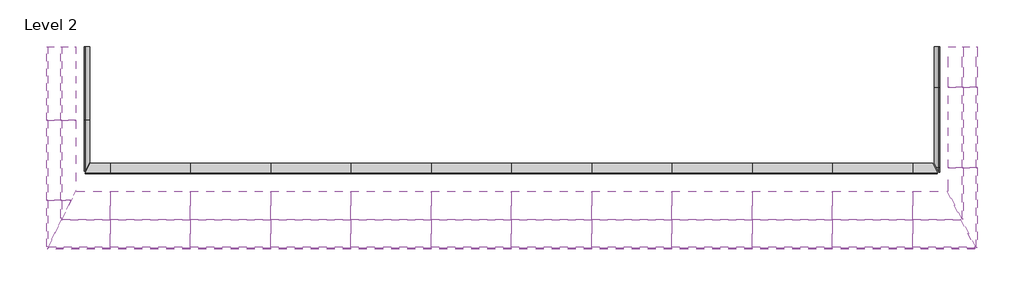
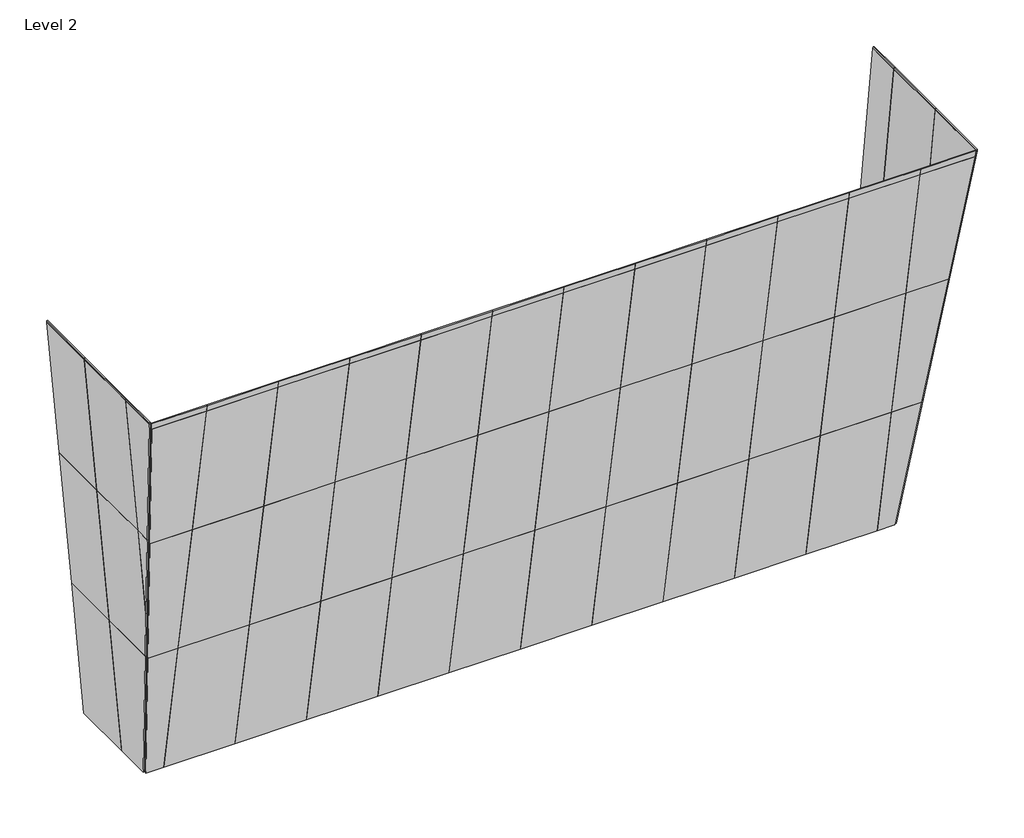
# One storey: 71 plates.
"""IFC4 building model written with IfcOpenShell, lengths in millimetres."""

import ifcopenshell
import ifcopenshell.guid

model = None  # the IFC model being written
_history = None  # IfcOwnerHistory: only IFC2X3 demands one
_inside = {}  # id of a spatial element -> (the spatial element, [elements in it])
_under = {}  # id of a project, library or spatial element -> (it, [spatial elements below it])
_declared = {}  # id of a project -> (the project, [libraries it declares])
_typed = {}  # id of a type object -> (the type object, [elements of that type])
_made_of = {}  # id of a material, layer set ... -> (it, [elements and type objects made of it])


def new_model(schema):
    """Start an empty IFC model of exactly this schema.

    Asked for "IFC4X3", IfcOpenShell would pick the latest addendum, in which some entities
    have other attributes; the version numbers below select the first issue.
    IFC2X3 requires an IfcOwnerHistory on every rooted entity: one is made here for all.
    """
    global model, _history
    if schema == "IFC4X3":
        model = ifcopenshell.file(schema_version=(4, 3, 0, 0))
    else:
        model = ifcopenshell.file(schema=schema)
    _inside.clear()
    _under.clear()
    _declared.clear()
    _typed.clear()
    _made_of.clear()
    _history = None
    if model.schema == "IFC2X3":
        org = make("IfcOrganization", Name="unknown")
        user = make(
            "IfcPersonAndOrganization",
            ThePerson=make("IfcPerson", FamilyName="unknown"),
            TheOrganization=org,
        )
        app = make(
            "IfcApplication",
            ApplicationDeveloper=org,
            Version="unknown",
            ApplicationFullName="unknown",
            ApplicationIdentifier="unknown",
        )
        _history = make(
            "IfcOwnerHistory",
            OwningUser=user,
            OwningApplication=app,
            ChangeAction="ADDED",
            CreationDate=0,
        )
    return model


def make(cls, **values):
    """One entity of the class cls with the attributes given. An attribute that is None is left unset."""
    return model.create_entity(
        cls, **{name: value for name, value in values.items() if value is not None}
    )


def rooted(cls, **values):
    """An entity with a GlobalId (a new one), such as an element, a storey or a relation."""
    return make(cls, GlobalId=ifcopenshell.guid.new(), OwnerHistory=_history, **values)


def si_unit(unit_type, name, prefix=None):
    """IfcSIUnit, for example si_unit("LENGTHUNIT", "METRE", prefix="MILLI")."""
    return make("IfcSIUnit", UnitType=unit_type, Prefix=prefix, Name=name)


def assignment(units):
    """IfcUnitAssignment: the units of a project."""
    return None if units is None else make("IfcUnitAssignment", Units=units)


def point(xyz):
    """IfcCartesianPoint."""
    return None if xyz is None else make("IfcCartesianPoint", Coordinates=xyz)


def direction(xyz):
    """IfcDirection."""
    return None if xyz is None else make("IfcDirection", DirectionRatios=xyz)


def frame(location, z_axis=None, x_axis=None):
    """IfcAxis2Placement3D, a coordinate frame: its origin and axes. An axis left out is left unset."""
    return make(
        "IfcAxis2Placement3D",
        Location=point(location),
        Axis=direction(z_axis),
        RefDirection=direction(x_axis),
    )


def origin():
    """The frame at (0, 0, 0) with its axes left unset."""
    return frame((0.0, 0.0, 0.0))


def origin_with_axes():
    """The frame at (0, 0, 0) with the z axis (0, 0, 1) and the x axis (1, 0, 0) written out."""
    return frame((0.0, 0.0, 0.0), z_axis=(0.0, 0.0, 1.0), x_axis=(1.0, 0.0, 0.0))


def place(relative_to, where):
    """IfcLocalPlacement: puts the frame where relative to a parent placement (None: the world)."""
    return make(
        "IfcLocalPlacement", PlacementRelTo=relative_to, RelativePlacement=where
    )


def context(
    kind, dimensions, precision=None, world=None, true_north=None, identifier=None
):
    """IfcGeometricRepresentationContext, for example the 3D "Model" context."""
    return make(
        "IfcGeometricRepresentationContext",
        ContextIdentifier=identifier,
        ContextType=kind,
        CoordinateSpaceDimension=dimensions,
        Precision=precision,
        WorldCoordinateSystem=world,
        TrueNorth=true_north,
    )


def project(units=None, contexts=None):
    """IfcProject with its units and contexts."""
    return rooted(
        "IfcProject",
        Name="project",
        RepresentationContexts=contexts,
        UnitsInContext=assignment(units),
    )


def spatial(cls, under=None, at=None, **own):
    """A site, building, storey or space (cls), placed at a placement, below another one or the project."""
    s = rooted(cls, ObjectPlacement=at, **own)
    if under is not None:
        _under.setdefault(under.id(), (under, []))[1].append(s)
    return s


def polyline(points):
    """IfcPolyline through the points."""
    return make("IfcPolyline", Points=[point(p) for p in points])


def outline(outer, holes=None, kind="AREA"):
    """IfcArbitraryClosedProfileDef: a profile drawn as a closed curve; with holes, ...WithVoids."""
    if holes is None:
        return make("IfcArbitraryClosedProfileDef", ProfileType=kind, OuterCurve=outer)
    return make(
        "IfcArbitraryProfileDefWithVoids",
        ProfileType=kind,
        OuterCurve=outer,
        InnerCurves=holes,
    )


def extrude(swept, where, along, depth):
    """IfcExtrudedAreaSolid: the profile swept, set in the frame where, extruded along a direction by depth."""
    return make(
        "IfcExtrudedAreaSolid",
        SweptArea=swept,
        Position=where,
        ExtrudedDirection=direction(along),
        Depth=depth,
    )


def shape(context_of_items, identifier, shape_type, items):
    """IfcShapeRepresentation: the items that make up one representation, for example the "Body"."""
    return make(
        "IfcShapeRepresentation",
        ContextOfItems=context_of_items,
        RepresentationIdentifier=identifier,
        RepresentationType=shape_type,
        Items=items,
    )


def source(mapping_origin, context_of_items, identifier, shape_type, items):
    """IfcRepresentationMap: a shape defined once, which mapped items show again and again."""
    return make(
        "IfcRepresentationMap",
        MappingOrigin=mapping_origin,
        MappedRepresentation=shape(context_of_items, identifier, shape_type, items),
    )


def transform(
    local_origin,
    x_axis=None,
    y_axis=None,
    z_axis=None,
    scale=None,
    scale2=None,
    scale3=None,
    uniform=True,
):
    """IfcCartesianTransformationOperator3D, or its non-uniform kind. x_axis, y_axis, z_axis: its Axis1, 2, 3."""
    if uniform:
        return make(
            "IfcCartesianTransformationOperator3D",
            Axis1=direction(x_axis),
            Axis2=direction(y_axis),
            LocalOrigin=point(local_origin),
            Scale=scale,
            Axis3=direction(z_axis),
        )
    return make(
        "IfcCartesianTransformationOperator3DnonUniform",
        Axis1=direction(x_axis),
        Axis2=direction(y_axis),
        LocalOrigin=point(local_origin),
        Scale=scale,
        Axis3=direction(z_axis),
        Scale2=scale2,
        Scale3=scale3,
    )


def mapped(mapping_source, mapping_target):
    """IfcMappedItem: shows the shape of a source again, moved by a transform."""
    return make(
        "IfcMappedItem", MappingSource=mapping_source, MappingTarget=mapping_target
    )


def made_of(thing, what):
    """Note that an element or type object is made of a material, layer set ...; save() writes the relation."""
    if what is not None:
        _made_of.setdefault(what.id(), (what, []))[1].append(thing)
    return thing


def element(
    cls,
    number,
    at=None,
    inside=None,
    cuts=None,
    type_object=None,
    material=None,
    context=None,
    identifier="Body",
    shape_type=None,
    held_by="IfcProductDefinitionShape",
    body=None,
    shapes=None,
    **own,
):
    """One element of the class cls, such as IfcWall. Its Tag is "e" and its number.

    at: its placement. inside: the storey or other place that contains it. cuts: it is an
    opening in that element (IfcRelVoidsElement). A single representation is given by context,
    identifier, shape_type and body (its items); several are given by shapes. held_by: the class
    of the entity that holds the representations. save() writes the other relations.
    """
    e = rooted(cls, Tag="e%d" % number, ObjectPlacement=at, **own)
    if body is not None:
        shapes = [shape(context, identifier, shape_type, body)]
    if shapes is not None:
        e.Representation = make(held_by, Representations=shapes)
    if inside is not None:
        _inside.setdefault(inside.id(), (inside, []))[1].append(e)
    if cuts is not None:
        rooted(
            "IfcRelVoidsElement", RelatingBuildingElement=cuts, RelatedOpeningElement=e
        )
    if type_object is not None:
        _typed.setdefault(type_object.id(), (type_object, []))[1].append(e)
    return made_of(e, material)


def aggregate(whole, parts):
    """IfcRelAggregates: a whole, such as a stair, and the parts it consists of."""
    return rooted("IfcRelAggregates", RelatingObject=whole, RelatedObjects=parts)


def save(model, path):
    """Write the relations noted so far, then the file.

    IfcRelAggregates (storeys below a building ...), IfcRelContainedInSpatialStructure (elements
    in a storey), IfcRelDefinesByType, IfcRelAssociatesMaterial and IfcRelDeclares: one each for
    every whole, place, type object, material and project.
    """
    for whole, parts in _under.values():
        aggregate(whole, parts)
    for where, things in _inside.values():
        rooted(
            "IfcRelContainedInSpatialStructure",
            RelatedElements=things,
            RelatingStructure=where,
        )
    for kind, things in _typed.values():
        rooted("IfcRelDefinesByType", RelatedObjects=things, RelatingType=kind)
    for what, things in _made_of.values():
        rooted("IfcRelAssociatesMaterial", RelatedObjects=things, RelatingMaterial=what)
    for by, libraries in _declared.values():
        rooted("IfcRelDeclares", RelatingContext=by, RelatedDefinitions=libraries)
    model.write(path)


def system_panel_glazed_2e91cb65(model_context):
    return source(origin(), model_context, "Body", "SweptSolid", [
        extrude(outline(polyline([(838.2000002, -44.45), (-838.2000002, -44.45), (-838.2000002, -19.05), (838.2000002, -19.05), (838.2000002, -44.45)])), origin_with_axes(), (0.0, 0.0, 1.0), 3657.6),
    ])


def system_panel_glazed_41c8569a(model_context):
    return source(origin(), model_context, "Body", "SweptSolid", [
        extrude(outline(polyline([(3054.1438606, -268.2393521), (0.0, 268.2393521), (3054.1438606, 268.2393521), (3054.1438606, -268.2393521)])), frame((0.0, -44.45, 0.0), z_axis=(0.0, 1.0, 0.0), x_axis=(0.0, 0.0, 1.0)), (0.0, 0.0, 1.0), 25.4),
    ])


def system_panel_glazed_2bad594a(model_context):
    return source(origin(), model_context, "Body", "SweptSolid", [
        extrude(outline(polyline([(0.0, -797.3917397), (0.0, 154.912342), (3657.6, 797.3917397), (3657.6, -797.3917397), (0.0, -797.3917397)])), frame((0.0, -44.45, 0.0), z_axis=(0.0, 1.0, 0.0), x_axis=(0.0, 0.0, 1.0)), (0.0, 0.0, 1.0), 25.4),
    ])


def system_panel_glazed_87679f4c(model_context):
    return source(origin(), model_context, "Body", "SweptSolid", [
        extrude(outline(polyline([(0.0, -914.4), (0.0, 680.3834794), (1332.2432262, 914.4), (3657.6, 914.4), (3657.6, -914.4), (0.0, -914.4)])), frame((0.0, -44.45, 0.0), z_axis=(0.0, 1.0, 0.0), x_axis=(0.0, 0.0, 1.0)), (0.0, 0.0, 1.0), 25.4),
    ])


def system_panel_glazed_96c5221b(model_context):
    return source(origin(), model_context, "Body", "SweptSolid", [
        extrude(outline(polyline([(0.0, -204.2314386), (2325.3567738, 204.2314386), (2325.3567738, -204.2314386), (0.0, -204.2314386)])), frame((0.0, -44.45, 0.0), z_axis=(0.0, 1.0, 0.0), x_axis=(0.0, 0.0, 1.0)), (0.0, 0.0, 1.0), 25.4),
    ])


def system_panel_glazed_1f34555f(model_context):
    return source(origin(), model_context, "Body", "SweptSolid", [
        extrude(outline(polyline([(914.4, -44.45), (-914.4, -44.45), (-914.4, -19.05), (914.4, -19.05), (914.4, -44.45)])), origin_with_axes(), (0.0, 0.0, 1.0), 3657.6),
    ])


def system_panel_glazed_ce152239(model_context):
    return source(origin(), model_context, "Body", "SweptSolid", [
        extrude(outline(polyline([(0.0, -525.4711374), (0.0, -117.0082603), (3657.6, 525.4711374), (3657.6, -525.4711374), (0.0, -525.4711374)])), frame((0.0, -44.45, 0.0), z_axis=(0.0, 1.0, 0.0), x_axis=(0.0, 0.0, 1.0)), (0.0, 0.0, 1.0), 25.4),
    ])


def system_panel_glazed_8b4ddac8(model_context):
    return source(origin(), model_context, "Body", "SweptSolid", [
        extrude(outline(polyline([(838.2000002, -44.45), (-838.2000002, -44.45), (-838.2000002, -19.05), (838.2000002, -19.05), (838.2000002, -44.45)])), origin_with_axes(), (0.0, 0.0, 1.0), 41.9143134),
    ])


def system_panel_glazed_7f82afe2(model_context):
    return source(origin(), model_context, "Body", "SweptSolid", [
        extrude(outline(polyline([(914.4, -44.45), (-914.4, -44.45), (-914.4, -19.05), (914.4, -19.05), (914.4, -44.45)])), origin_with_axes(), (0.0, 0.0, 1.0), 41.9143134),
    ])


def system_panel_glazed_3146f186(model_context):
    return source(origin(), model_context, "Body", "SweptSolid", [
        extrude(outline(polyline([(0.0, -529.1523878), (0.0, 521.789887), (41.9143134, 529.1523878), (41.9143134, -529.1523878), (0.0, -529.1523878)])), frame((0.0, -44.45, 0.0), z_axis=(0.0, 1.0, 0.0), x_axis=(0.0, 0.0, 1.0)), (0.0, 0.0, 1.0), 25.4),
    ])


def system_panel_glazed_f4345ae3(model_context):
    return source(origin(), model_context, "Body", "SweptSolid", [
        extrude(outline(polyline([(914.4, -44.45), (-914.4, -44.45), (-914.4, -19.05), (914.4, -19.05), (914.4, -44.45)])), origin_with_axes(), (0.0, 0.0, 1.0), 169.2731269),
    ])


def system_panel_glazed_866ab655(model_context):
    return source(origin(), model_context, "Body", "SweptSolid", [
        extrude(outline(polyline([(0.0, -808.3993064), (0.0, 914.4), (3657.6, 914.4), (3657.6, -914.4), (603.4561394, -914.4), (0.0, -808.3993064)])), frame((0.0, -44.45, 0.0), z_axis=(0.0, 1.0, 0.0), x_axis=(0.0, 0.0, 1.0)), (0.0, 0.0, 1.0), 25.4),
    ])


def system_panel_glazed_b062bbc2(model_context):
    return source(origin(), model_context, "Body", "SweptSolid", [
        extrude(outline(polyline([(465.8483058, -44.45), (-465.8483058, -44.45), (-465.8483058, -19.05), (465.8483058, -19.05), (465.8483058, -44.45)])), origin_with_axes(), (0.0, 0.0, 1.0), 3657.6),
    ])


def system_panel_glazed_bcd6892e(model_context):
    return source(origin(), model_context, "Body", "SweptSolid", [
        extrude(outline(polyline([(0.0, 53.0003468), (0.0, 589.4790509), (3657.6, 589.4790509), (3657.6, -589.4790509), (0.0, 53.0003468)])), frame((0.0, -44.45, 0.0), z_axis=(0.0, 1.0, 0.0), x_axis=(0.0, 0.0, 1.0)), (0.0, 0.0, 1.0), 25.4),
    ])


def system_panel_glazed_e7bd2299(model_context):
    return source(origin(), model_context, "Body", "SweptSolid", [
        extrude(outline(polyline([(0.0, -268.2393521), (0.0, 910.7187498), (3657.6, 910.7187498), (3657.6, -910.7187498), (0.0, -268.2393521)])), frame((0.0, -44.45, 0.0), z_axis=(0.0, 1.0, 0.0), x_axis=(0.0, 0.0, 1.0)), (0.0, 0.0, 1.0), 25.4),
    ])


def system_panel_glazed_0a43eb3e(model_context):
    return source(origin(), model_context, "Body", "SweptSolid", [
        extrude(outline(polyline([(0.0, -907.0374994), (0.0, 914.4000002), (41.9143134, 914.4000002), (41.9143134, -914.4000002), (0.0, -907.0374994)])), frame((0.0, -44.45, 0.0), z_axis=(0.0, 1.0, 0.0), x_axis=(0.0, 0.0, 1.0)), (0.0, 0.0, 1.0), 25.4),
    ])


def system_panel_glazed_c48c36d0(model_context):
    return source(origin(), model_context, "Body", "SweptSolid", [
        extrude(outline(polyline([(465.8483058, -44.45), (-465.8483058, -44.45), (-465.8483058, -19.05), (465.8483058, -19.05), (465.8483058, -44.45)])), origin_with_axes(), (0.0, 0.0, 1.0), 41.9143134),
    ])


def system_panel_glazed_35afb83b(model_context):
    return source(origin(), model_context, "Body", "SweptSolid", [
        extrude(outline(polyline([(0.0, -71.0314805), (0.0, 386.1685195), (3657.6, 386.1685195), (3657.6, -386.1685195), (0.0, -71.0314805)])), frame((0.0, -44.45, 0.0), z_axis=(0.0, 1.0, 0.0), x_axis=(0.0, 0.0, 1.0)), (0.0, 0.0, 1.0), 25.4),
    ])


def system_panel_glazed_ca25d662(model_context):
    return source(origin(), model_context, "Body", "SweptSolid", [
        extrude(outline(polyline([(0.0, -386.1685195), (0.0, 71.0314805), (3657.6, 386.1685195), (3657.6, -386.1685195), (0.0, -386.1685195)])), frame((0.0, -44.45, 0.0), z_axis=(0.0, 1.0, 0.0), x_axis=(0.0, 0.0, 1.0)), (0.0, 0.0, 1.0), 25.4),
    ])


def system_panel_glazed_d5b9b34d(model_context):
    return source(origin(), model_context, "Body", "SweptSolid", [
        extrude(outline(polyline([(0.0, -228.6), (0.0, 543.7370389), (3657.6, 543.7370389), (3657.6, -543.7370389), (0.0, -228.6)])), frame((0.0, -44.45, 0.0), z_axis=(0.0, 1.0, 0.0), x_axis=(0.0, 0.0, 1.0)), (0.0, 0.0, 1.0), 25.4),
    ])


def system_panel_glazed_127879aa(model_context):
    return source(origin(), model_context, "Body", "SweptSolid", [
        extrude(outline(polyline([(0.0, -543.7370389), (0.0, 228.6), (3657.6, 543.7370389), (3657.6, -543.7370389), (0.0, -543.7370389)])), frame((0.0, -44.45, 0.0), z_axis=(0.0, 1.0, 0.0), x_axis=(0.0, 0.0, 1.0)), (0.0, 0.0, 1.0), 25.4),
    ])


def system_panel_glazed_cde5e94a(model_context):
    return source(origin(), model_context, "Body", "SweptSolid", [
        extrude(outline(polyline([(0.0, -386.1685195), (0.0, 701.3055584), (3657.6, 701.3055584), (3657.6, -701.3055584), (0.0, -386.1685195)])), frame((0.0, -44.45, 0.0), z_axis=(0.0, 1.0, 0.0), x_axis=(0.0, 0.0, 1.0)), (0.0, 0.0, 1.0), 25.4),
    ])


def system_panel_glazed_b3fa7013(model_context):
    return source(origin(), model_context, "Body", "SweptSolid", [
        extrude(outline(polyline([(0.0, -701.3055584), (0.0, 386.1685195), (3657.6, 701.3055584), (3657.6, -701.3055584), (0.0, -701.3055584)])), frame((0.0, -44.45, 0.0), z_axis=(0.0, 1.0, 0.0), x_axis=(0.0, 0.0, 1.0)), (0.0, 0.0, 1.0), 25.4),
    ])


def system_panel_glazed_d86b06c2(model_context):
    return source(origin(), model_context, "Body", "SweptSolid", [
        extrude(outline(polyline([(0.0, -694.0133132), (0.0, 708.5978036), (169.2731269, 708.5978036), (169.2731269, -708.5978036), (0.0, -694.0133132)])), frame((0.0, -44.45, 0.0), z_axis=(0.0, 1.0, 0.0), x_axis=(0.0, 0.0, 1.0)), (0.0, 0.0, 1.0), 25.4),
    ])


def system_panel_glazed_9c30f1a4(model_context):
    return source(origin(), model_context, "Body", "SweptSolid", [
        extrude(outline(polyline([(0.0, -708.5978036), (0.0, 694.0133132), (169.2731269, 708.5978036), (169.2731269, -708.5978036), (0.0, -708.5978036)])), frame((0.0, -44.45, 0.0), z_axis=(0.0, 1.0, 0.0), x_axis=(0.0, 0.0, 1.0)), (0.0, 0.0, 1.0), 25.4),
    ])


model = new_model("IFC4")

# Units and contexts
model_context = context("Model", 3, world=origin())
ifc_project = project(units=[si_unit("LENGTHUNIT", "METRE", prefix="MILLI")], contexts=[model_context])

# Site, building, storey
site = spatial("IfcSite", under=ifc_project)
building = spatial("IfcBuilding", under=site)
storey = spatial("IfcBuildingStorey", under=building, Name="Level 2", Elevation=3657.6)

# Plates
placement = place(None, origin())
system_panel_glazed_shape = system_panel_glazed_2e91cb65(model_context)
element("IfcPlate", 1, ObjectType="System Panel : Glazed", at=placement, inside=storey, context=model_context, shape_type="MappedRepresentation", body=[
    mapped(system_panel_glazed_shape, transform((-10766.9154339, -10749.0984697, 3656.4931221), x_axis=(0.0, -1.0, 0.0), y_axis=(0.9961946980917455, 0.0, 0.08715574274765803), z_axis=(-0.08715574274765803, 0.0, 0.9961946980917455))),
])
element("IfcPlate", 2, ObjectType="System Panel : Glazed", at=placement, inside=storey, context=model_context, shape_type="MappedRepresentation", body=[
    mapped(system_panel_glazed_shape, transform((-11085.6962786, -10749.0984697, 7300.1748498), x_axis=(0.0, -1.0, 0.0), y_axis=(0.9961946980917455, 0.0, 0.08715574274765803), z_axis=(-0.08715574274765803, 0.0, 0.9961946980917455))),
])
element("IfcPlate", 3, ObjectType="System Panel : Glazed", at=placement, inside=storey, context=model_context, shape_type="MappedRepresentation", body=[
    mapped(system_panel_glazed_shape, transform((-11404.4771233, -10749.0984697, 10943.8565775), x_axis=(0.0, -1.0, 0.0), y_axis=(0.9961946980917455, 0.0, 0.08715574274765803), z_axis=(-0.08715574274765803, 0.0, 0.9961946980917455))),
])
system_panel_glazed_2_shape = system_panel_glazed_41c8569a(model_context)
element("IfcPlate", 4, ObjectType="System Panel : Glazed", at=placement, inside=storey, context=model_context, shape_type="MappedRepresentation", body=[
    mapped(system_panel_glazed_2_shape, transform((8487.8855556, -12939.6344332, 4257.6529286), x_axis=(0.0, 1.0, 0.0), y_axis=(-0.9961946980917455, 0.0, 0.08715574274765803), z_axis=(0.08715574274765803, 0.0, 0.9961946980917455))),
])
system_panel_glazed_3_shape = system_panel_glazed_2bad594a(model_context)
element("IfcPlate", 5, ObjectType="System Panel : Glazed", at=placement, inside=storey, context=model_context, shape_type="MappedRepresentation", body=[
    mapped(system_panel_glazed_3_shape, transform((-10766.9154339, -12384.6902096, 3656.4931221), x_axis=(0.0, -1.0, 0.0), y_axis=(0.9961946980917455, 0.0, 0.08715574274765803), z_axis=(-0.08715574274765803, 0.0, 0.9961946980917455))),
])
system_panel_glazed_4_shape = system_panel_glazed_87679f4c(model_context)
element("IfcPlate", 6, ObjectType="System Panel : Glazed", at=placement, inside=storey, context=model_context, shape_type="MappedRepresentation", body=[
    mapped(system_panel_glazed_4_shape, transform((-11085.6962786, -12501.6984699, 7300.1748498), x_axis=(0.0, -1.0, 0.0), y_axis=(0.9961946980917455, 0.0, 0.08715574274765803), z_axis=(-0.08715574274765803, 0.0, 0.9961946980917455))),
])
system_panel_glazed_5_shape = system_panel_glazed_96c5221b(model_context)
element("IfcPlate", 7, ObjectType="System Panel : Glazed", at=placement, inside=storey, context=model_context, shape_type="MappedRepresentation", body=[
    mapped(system_panel_glazed_5_shape, transform((-11201.8089265, -13620.3299085, 8627.3484884), x_axis=(0.0, -1.0, 0.0), y_axis=(0.9961946980917455, 0.0, 0.08715574274765803), z_axis=(-0.08715574274765803, 0.0, 0.9961946980917455))),
])
system_panel_glazed_6_shape = system_panel_glazed_1f34555f(model_context)
element("IfcPlate", 8, ObjectType="System Panel : Glazed", at=placement, inside=storey, context=model_context, shape_type="MappedRepresentation", body=[
    mapped(system_panel_glazed_6_shape, transform((-11404.4771233, -12501.6984699, 10943.8565775), x_axis=(0.0, -1.0, 0.0), y_axis=(0.9961946980917455, 0.0, 0.08715574274765803), z_axis=(-0.08715574274765803, 0.0, 0.9961946980917455))),
])
element("IfcPlate", 9, ObjectType="System Panel : Glazed", at=placement, inside=storey, context=model_context, shape_type="MappedRepresentation", body=[
    mapped(system_panel_glazed_6_shape, transform((-9408.1607851, -12552.1096101, 3655.3946681), x_axis=(1.0, 0.0, 0.0), y_axis=(0.0, 0.9848077530122081, 0.17364817766693014), z_axis=(0.0, -0.17364817766693014, 0.9848077530122081))),
])
element("IfcPlate", 10, ObjectType="System Panel : Glazed", at=placement, inside=storey, context=model_context, shape_type="MappedRepresentation", body=[
    mapped(system_panel_glazed_6_shape, transform((-7579.3607851, -12552.1096101, 3655.3946681), x_axis=(1.0, 0.0, 0.0), y_axis=(0.0, 0.9848077530122081, 0.17364817766693014), z_axis=(0.0, -0.17364817766693014, 0.9848077530122081))),
])
element("IfcPlate", 11, ObjectType="System Panel : Glazed", at=placement, inside=storey, context=model_context, shape_type="MappedRepresentation", body=[
    mapped(system_panel_glazed_6_shape, transform((-5750.5607851, -12552.1096101, 3655.3946681), x_axis=(1.0, 0.0, 0.0), y_axis=(0.0, 0.9848077530122081, 0.17364817766693014), z_axis=(0.0, -0.17364817766693014, 0.9848077530122081))),
])
element("IfcPlate", 12, ObjectType="System Panel : Glazed", at=placement, inside=storey, context=model_context, shape_type="MappedRepresentation", body=[
    mapped(system_panel_glazed_6_shape, transform((-3921.7607851, -12552.1096101, 3655.3946681), x_axis=(1.0, 0.0, 0.0), y_axis=(0.0, 0.9848077530122081, 0.17364817766693014), z_axis=(0.0, -0.17364817766693014, 0.9848077530122081))),
])
element("IfcPlate", 13, ObjectType="System Panel : Glazed", at=placement, inside=storey, context=model_context, shape_type="MappedRepresentation", body=[
    mapped(system_panel_glazed_6_shape, transform((-2092.9607851, -12552.1096101, 3655.3946681), x_axis=(1.0, 0.0, 0.0), y_axis=(0.0, 0.9848077530122081, 0.17364817766693014), z_axis=(0.0, -0.17364817766693014, 0.9848077530122081))),
])
element("IfcPlate", 14, ObjectType="System Panel : Glazed", at=placement, inside=storey, context=model_context, shape_type="MappedRepresentation", body=[
    mapped(system_panel_glazed_6_shape, transform((-264.1607851, -12552.1096101, 3655.3946681), x_axis=(1.0, 0.0, 0.0), y_axis=(0.0, 0.9848077530122081, 0.17364817766693014), z_axis=(0.0, -0.17364817766693014, 0.9848077530122081))),
])
element("IfcPlate", 15, ObjectType="System Panel : Glazed", at=placement, inside=storey, context=model_context, shape_type="MappedRepresentation", body=[
    mapped(system_panel_glazed_6_shape, transform((1564.6392149, -12552.1096101, 3655.3946681), x_axis=(1.0, 0.0, 0.0), y_axis=(0.0, 0.9848077530122081, 0.17364817766693014), z_axis=(0.0, -0.17364817766693014, 0.9848077530122081))),
])
element("IfcPlate", 16, ObjectType="System Panel : Glazed", at=placement, inside=storey, context=model_context, shape_type="MappedRepresentation", body=[
    mapped(system_panel_glazed_6_shape, transform((3393.4392149, -12552.1096101, 3655.3946681), x_axis=(1.0, 0.0, 0.0), y_axis=(0.0, 0.9848077530122081, 0.17364817766693014), z_axis=(0.0, -0.17364817766693014, 0.9848077530122081))),
])
element("IfcPlate", 17, ObjectType="System Panel : Glazed", at=placement, inside=storey, context=model_context, shape_type="MappedRepresentation", body=[
    mapped(system_panel_glazed_6_shape, transform((5222.2392149, -12552.1096101, 3655.3946681), x_axis=(1.0, 0.0, 0.0), y_axis=(0.0, 0.9848077530122081, 0.17364817766693014), z_axis=(0.0, -0.17364817766693014, 0.9848077530122081))),
])
element("IfcPlate", 18, ObjectType="System Panel : Glazed", at=placement, inside=storey, context=model_context, shape_type="MappedRepresentation", body=[
    mapped(system_panel_glazed_6_shape, transform((7051.0392149, -12552.1096101, 3655.3946681), x_axis=(1.0, 0.0, 0.0), y_axis=(0.0, 0.9848077530122081, 0.17364817766693014), z_axis=(0.0, -0.17364817766693014, 0.9848077530122081))),
])
element("IfcPlate", 19, ObjectType="System Panel : Glazed", at=placement, inside=storey, context=model_context, shape_type="MappedRepresentation", body=[
    mapped(system_panel_glazed_6_shape, transform((-9408.1607851, -13187.2451847, 7257.4275056), x_axis=(1.0, 0.0, 0.0), y_axis=(0.0, 0.9848077530122081, 0.17364817766693014), z_axis=(0.0, -0.17364817766693014, 0.9848077530122081))),
])
element("IfcPlate", 20, ObjectType="System Panel : Glazed", at=placement, inside=storey, context=model_context, shape_type="MappedRepresentation", body=[
    mapped(system_panel_glazed_6_shape, transform((-7579.3607851, -13187.2451847, 7257.4275056), x_axis=(1.0, 0.0, 0.0), y_axis=(0.0, 0.9848077530122081, 0.17364817766693014), z_axis=(0.0, -0.17364817766693014, 0.9848077530122081))),
])
element("IfcPlate", 21, ObjectType="System Panel : Glazed", at=placement, inside=storey, context=model_context, shape_type="MappedRepresentation", body=[
    mapped(system_panel_glazed_6_shape, transform((-5750.5607851, -13187.2451847, 7257.4275056), x_axis=(1.0, 0.0, 0.0), y_axis=(0.0, 0.9848077530122081, 0.17364817766693014), z_axis=(0.0, -0.17364817766693014, 0.9848077530122081))),
])
element("IfcPlate", 22, ObjectType="System Panel : Glazed", at=placement, inside=storey, context=model_context, shape_type="MappedRepresentation", body=[
    mapped(system_panel_glazed_6_shape, transform((-3921.7607851, -13187.2451847, 7257.4275056), x_axis=(1.0, 0.0, 0.0), y_axis=(0.0, 0.9848077530122081, 0.17364817766693014), z_axis=(0.0, -0.17364817766693014, 0.9848077530122081))),
])
element("IfcPlate", 23, ObjectType="System Panel : Glazed", at=placement, inside=storey, context=model_context, shape_type="MappedRepresentation", body=[
    mapped(system_panel_glazed_6_shape, transform((-2092.9607851, -13187.2451847, 7257.4275056), x_axis=(1.0, 0.0, 0.0), y_axis=(0.0, 0.9848077530122081, 0.17364817766693014), z_axis=(0.0, -0.17364817766693014, 0.9848077530122081))),
])
element("IfcPlate", 24, ObjectType="System Panel : Glazed", at=placement, inside=storey, context=model_context, shape_type="MappedRepresentation", body=[
    mapped(system_panel_glazed_6_shape, transform((-264.1607851, -13187.2451847, 7257.4275056), x_axis=(1.0, 0.0, 0.0), y_axis=(0.0, 0.9848077530122081, 0.17364817766693014), z_axis=(0.0, -0.17364817766693014, 0.9848077530122081))),
])
element("IfcPlate", 25, ObjectType="System Panel : Glazed", at=placement, inside=storey, context=model_context, shape_type="MappedRepresentation", body=[
    mapped(system_panel_glazed_6_shape, transform((1564.6392149, -13187.2451847, 7257.4275056), x_axis=(1.0, 0.0, 0.0), y_axis=(0.0, 0.9848077530122081, 0.17364817766693014), z_axis=(0.0, -0.17364817766693014, 0.9848077530122081))),
])
element("IfcPlate", 26, ObjectType="System Panel : Glazed", at=placement, inside=storey, context=model_context, shape_type="MappedRepresentation", body=[
    mapped(system_panel_glazed_6_shape, transform((3393.4392149, -13187.2451847, 7257.4275056), x_axis=(1.0, 0.0, 0.0), y_axis=(0.0, 0.9848077530122081, 0.17364817766693014), z_axis=(0.0, -0.17364817766693014, 0.9848077530122081))),
])
element("IfcPlate", 27, ObjectType="System Panel : Glazed", at=placement, inside=storey, context=model_context, shape_type="MappedRepresentation", body=[
    mapped(system_panel_glazed_6_shape, transform((5222.2392149, -13187.2451847, 7257.4275056), x_axis=(1.0, 0.0, 0.0), y_axis=(0.0, 0.9848077530122081, 0.17364817766693014), z_axis=(0.0, -0.17364817766693014, 0.9848077530122081))),
])
element("IfcPlate", 28, ObjectType="System Panel : Glazed", at=placement, inside=storey, context=model_context, shape_type="MappedRepresentation", body=[
    mapped(system_panel_glazed_6_shape, transform((7051.0392149, -13187.2451847, 7257.4275056), x_axis=(1.0, 0.0, 0.0), y_axis=(0.0, 0.9848077530122081, 0.17364817766693014), z_axis=(0.0, -0.17364817766693014, 0.9848077530122081))),
])
element("IfcPlate", 29, ObjectType="System Panel : Glazed", at=placement, inside=storey, context=model_context, shape_type="MappedRepresentation", body=[
    mapped(system_panel_glazed_6_shape, transform((-9408.1607851, -13822.3807593, 10859.460343), x_axis=(1.0, 0.0, 0.0), y_axis=(0.0, 0.9848077530122081, 0.17364817766693014), z_axis=(0.0, -0.17364817766693014, 0.9848077530122081))),
])
element("IfcPlate", 30, ObjectType="System Panel : Glazed", at=placement, inside=storey, context=model_context, shape_type="MappedRepresentation", body=[
    mapped(system_panel_glazed_6_shape, transform((-7579.3607851, -13822.3807593, 10859.460343), x_axis=(1.0, 0.0, 0.0), y_axis=(0.0, 0.9848077530122081, 0.17364817766693014), z_axis=(0.0, -0.17364817766693014, 0.9848077530122081))),
])
element("IfcPlate", 31, ObjectType="System Panel : Glazed", at=placement, inside=storey, context=model_context, shape_type="MappedRepresentation", body=[
    mapped(system_panel_glazed_6_shape, transform((-5750.5607851, -13822.3807593, 10859.460343), x_axis=(1.0, 0.0, 0.0), y_axis=(0.0, 0.9848077530122081, 0.17364817766693014), z_axis=(0.0, -0.17364817766693014, 0.9848077530122081))),
])
element("IfcPlate", 32, ObjectType="System Panel : Glazed", at=placement, inside=storey, context=model_context, shape_type="MappedRepresentation", body=[
    mapped(system_panel_glazed_6_shape, transform((-3921.7607851, -13822.3807593, 10859.460343), x_axis=(1.0, 0.0, 0.0), y_axis=(0.0, 0.9848077530122081, 0.17364817766693014), z_axis=(0.0, -0.17364817766693014, 0.9848077530122081))),
])
element("IfcPlate", 33, ObjectType="System Panel : Glazed", at=placement, inside=storey, context=model_context, shape_type="MappedRepresentation", body=[
    mapped(system_panel_glazed_6_shape, transform((-2092.9607851, -13822.3807593, 10859.460343), x_axis=(1.0, 0.0, 0.0), y_axis=(0.0, 0.9848077530122081, 0.17364817766693014), z_axis=(0.0, -0.17364817766693014, 0.9848077530122081))),
])
element("IfcPlate", 34, ObjectType="System Panel : Glazed", at=placement, inside=storey, context=model_context, shape_type="MappedRepresentation", body=[
    mapped(system_panel_glazed_6_shape, transform((-264.1607851, -13822.3807593, 10859.460343), x_axis=(1.0, 0.0, 0.0), y_axis=(0.0, 0.9848077530122081, 0.17364817766693014), z_axis=(0.0, -0.17364817766693014, 0.9848077530122081))),
])
element("IfcPlate", 35, ObjectType="System Panel : Glazed", at=placement, inside=storey, context=model_context, shape_type="MappedRepresentation", body=[
    mapped(system_panel_glazed_6_shape, transform((1564.6392149, -13822.3807593, 10859.460343), x_axis=(1.0, 0.0, 0.0), y_axis=(0.0, 0.9848077530122081, 0.17364817766693014), z_axis=(0.0, -0.17364817766693014, 0.9848077530122081))),
])
element("IfcPlate", 36, ObjectType="System Panel : Glazed", at=placement, inside=storey, context=model_context, shape_type="MappedRepresentation", body=[
    mapped(system_panel_glazed_6_shape, transform((3393.4392149, -13822.3807593, 10859.460343), x_axis=(1.0, 0.0, 0.0), y_axis=(0.0, 0.9848077530122081, 0.17364817766693014), z_axis=(0.0, -0.17364817766693014, 0.9848077530122081))),
])
element("IfcPlate", 37, ObjectType="System Panel : Glazed", at=placement, inside=storey, context=model_context, shape_type="MappedRepresentation", body=[
    mapped(system_panel_glazed_6_shape, transform((5222.2392149, -13822.3807593, 10859.460343), x_axis=(1.0, 0.0, 0.0), y_axis=(0.0, 0.9848077530122081, 0.17364817766693014), z_axis=(0.0, -0.17364817766693014, 0.9848077530122081))),
])
element("IfcPlate", 38, ObjectType="System Panel : Glazed", at=placement, inside=storey, context=model_context, shape_type="MappedRepresentation", body=[
    mapped(system_panel_glazed_6_shape, transform((7051.0392149, -13822.3807593, 10859.460343), x_axis=(1.0, 0.0, 0.0), y_axis=(0.0, 0.9848077530122081, 0.17364817766693014), z_axis=(0.0, -0.17364817766693014, 0.9848077530122081))),
])
element("IfcPlate", 39, ObjectType="System Panel : Glazed", at=placement, inside=storey, context=model_context, shape_type="MappedRepresentation", body=[
    mapped(system_panel_glazed_6_shape, transform((8754.0717322, -11756.9950812, 7300.1748498), x_axis=(0.0, 1.0, 0.0), y_axis=(-0.9961946980917455, 0.0, 0.08715574274765803), z_axis=(0.08715574274765803, 0.0, 0.9961946980917455))),
])
element("IfcPlate", 40, ObjectType="System Panel : Glazed", at=placement, inside=storey, context=model_context, shape_type="MappedRepresentation", body=[
    mapped(system_panel_glazed_6_shape, transform((9072.8525769, -11756.9950812, 10943.8565775), x_axis=(0.0, 1.0, 0.0), y_axis=(-0.9961946980917455, 0.0, 0.08715574274765803), z_axis=(0.08715574274765803, 0.0, 0.9961946980917455))),
])
system_panel_glazed_7_shape = system_panel_glazed_ce152239(model_context)
element("IfcPlate", 41, ObjectType="System Panel : Glazed", at=placement, inside=storey, context=model_context, shape_type="MappedRepresentation", body=[
    mapped(system_panel_glazed_7_shape, transform((-11404.4771233, -13941.5696073, 10943.8565775), x_axis=(0.0, -1.0, 0.0), y_axis=(0.9961946980917455, 0.0, 0.08715574274765803), z_axis=(-0.08715574274765803, 0.0, 0.9961946980917455))),
])
system_panel_glazed_8_shape = system_panel_glazed_8b4ddac8(model_context)
element("IfcPlate", 42, ObjectType="System Panel : Glazed", at=placement, inside=storey, context=model_context, shape_type="MappedRepresentation", body=[
    mapped(system_panel_glazed_8_shape, transform((-11723.2579679, -10749.0984697, 14587.5383053), x_axis=(0.0, -1.0, 0.0), y_axis=(0.9961946980917455, 0.0, 0.08715574274765803), z_axis=(-0.08715574274765803, 0.0, 0.9961946980917455))),
])
system_panel_glazed_9_shape = system_panel_glazed_7f82afe2(model_context)
element("IfcPlate", 43, ObjectType="System Panel : Glazed", at=placement, inside=storey, context=model_context, shape_type="MappedRepresentation", body=[
    mapped(system_panel_glazed_9_shape, transform((-11723.2579679, -12501.6984699, 14587.5383053), x_axis=(0.0, -1.0, 0.0), y_axis=(0.9961946980917455, 0.0, 0.08715574274765803), z_axis=(-0.08715574274765803, 0.0, 0.9961946980917455))),
])
element("IfcPlate", 44, ObjectType="System Panel : Glazed", at=placement, inside=storey, context=model_context, shape_type="MappedRepresentation", body=[
    mapped(system_panel_glazed_9_shape, transform((9391.6334216, -11756.9950812, 14587.5383053), x_axis=(0.0, 1.0, 0.0), y_axis=(-0.9961946980917455, 0.0, 0.08715574274765803), z_axis=(0.08715574274765803, 0.0, 0.9961946980917455))),
])
system_panel_glazed_10_shape = system_panel_glazed_3146f186(model_context)
element("IfcPlate", 45, ObjectType="System Panel : Glazed", at=placement, inside=storey, context=model_context, shape_type="MappedRepresentation", body=[
    mapped(system_panel_glazed_10_shape, transform((-11723.2579679, -13945.2508577, 14587.5383053), x_axis=(0.0, -1.0, 0.0), y_axis=(0.9961946980917455, 0.0, 0.08715574274765803), z_axis=(-0.08715574274765803, 0.0, 0.9961946980917455))),
])
system_panel_glazed_11_shape = system_panel_glazed_f4345ae3(model_context)
element("IfcPlate", 46, ObjectType="System Panel : Glazed", at=placement, inside=storey, context=model_context, shape_type="MappedRepresentation", body=[
    mapped(system_panel_glazed_11_shape, transform((-9408.1607851, -14457.516334, 14461.4931804), x_axis=(1.0, 0.0, 0.0), y_axis=(0.0, 0.9848077530122081, 0.17364817766693014), z_axis=(0.0, -0.17364817766693014, 0.9848077530122081))),
])
element("IfcPlate", 47, ObjectType="System Panel : Glazed", at=placement, inside=storey, context=model_context, shape_type="MappedRepresentation", body=[
    mapped(system_panel_glazed_11_shape, transform((-7579.3607851, -14457.516334, 14461.4931804), x_axis=(1.0, 0.0, 0.0), y_axis=(0.0, 0.9848077530122081, 0.17364817766693014), z_axis=(0.0, -0.17364817766693014, 0.9848077530122081))),
])
element("IfcPlate", 48, ObjectType="System Panel : Glazed", at=placement, inside=storey, context=model_context, shape_type="MappedRepresentation", body=[
    mapped(system_panel_glazed_11_shape, transform((-5750.5607851, -14457.516334, 14461.4931804), x_axis=(1.0, 0.0, 0.0), y_axis=(0.0, 0.9848077530122081, 0.17364817766693014), z_axis=(0.0, -0.17364817766693014, 0.9848077530122081))),
])
element("IfcPlate", 49, ObjectType="System Panel : Glazed", at=placement, inside=storey, context=model_context, shape_type="MappedRepresentation", body=[
    mapped(system_panel_glazed_11_shape, transform((-3921.7607851, -14457.516334, 14461.4931804), x_axis=(1.0, 0.0, 0.0), y_axis=(0.0, 0.9848077530122081, 0.17364817766693014), z_axis=(0.0, -0.17364817766693014, 0.9848077530122081))),
])
element("IfcPlate", 50, ObjectType="System Panel : Glazed", at=placement, inside=storey, context=model_context, shape_type="MappedRepresentation", body=[
    mapped(system_panel_glazed_11_shape, transform((-2092.9607851, -14457.516334, 14461.4931804), x_axis=(1.0, 0.0, 0.0), y_axis=(0.0, 0.9848077530122081, 0.17364817766693014), z_axis=(0.0, -0.17364817766693014, 0.9848077530122081))),
])
element("IfcPlate", 51, ObjectType="System Panel : Glazed", at=placement, inside=storey, context=model_context, shape_type="MappedRepresentation", body=[
    mapped(system_panel_glazed_11_shape, transform((-264.1607851, -14457.516334, 14461.4931804), x_axis=(1.0, 0.0, 0.0), y_axis=(0.0, 0.9848077530122081, 0.17364817766693014), z_axis=(0.0, -0.17364817766693014, 0.9848077530122081))),
])
element("IfcPlate", 52, ObjectType="System Panel : Glazed", at=placement, inside=storey, context=model_context, shape_type="MappedRepresentation", body=[
    mapped(system_panel_glazed_11_shape, transform((1564.6392149, -14457.516334, 14461.4931804), x_axis=(1.0, 0.0, 0.0), y_axis=(0.0, 0.9848077530122081, 0.17364817766693014), z_axis=(0.0, -0.17364817766693014, 0.9848077530122081))),
])
element("IfcPlate", 53, ObjectType="System Panel : Glazed", at=placement, inside=storey, context=model_context, shape_type="MappedRepresentation", body=[
    mapped(system_panel_glazed_11_shape, transform((3393.4392149, -14457.516334, 14461.4931804), x_axis=(1.0, 0.0, 0.0), y_axis=(0.0, 0.9848077530122081, 0.17364817766693014), z_axis=(0.0, -0.17364817766693014, 0.9848077530122081))),
])
element("IfcPlate", 54, ObjectType="System Panel : Glazed", at=placement, inside=storey, context=model_context, shape_type="MappedRepresentation", body=[
    mapped(system_panel_glazed_11_shape, transform((5222.2392149, -14457.516334, 14461.4931804), x_axis=(1.0, 0.0, 0.0), y_axis=(0.0, 0.9848077530122081, 0.17364817766693014), z_axis=(0.0, -0.17364817766693014, 0.9848077530122081))),
])
element("IfcPlate", 55, ObjectType="System Panel : Glazed", at=placement, inside=storey, context=model_context, shape_type="MappedRepresentation", body=[
    mapped(system_panel_glazed_11_shape, transform((7051.0392149, -14457.516334, 14461.4931804), x_axis=(1.0, 0.0, 0.0), y_axis=(0.0, 0.9848077530122081, 0.17364817766693014), z_axis=(0.0, -0.17364817766693014, 0.9848077530122081))),
])
system_panel_glazed_12_shape = system_panel_glazed_866ab655(model_context)
element("IfcPlate", 56, ObjectType="System Panel : Glazed", at=placement, inside=storey, context=model_context, shape_type="MappedRepresentation", body=[
    mapped(system_panel_glazed_12_shape, transform((8435.2908875, -11756.9950812, 3656.4931221), x_axis=(0.0, 1.0, 0.0), y_axis=(-0.9961946980917455, 0.0, 0.08715574274765803), z_axis=(0.08715574274765803, 0.0, 0.9961946980917455))),
])
system_panel_glazed_13_shape = system_panel_glazed_b062bbc2(model_context)
element("IfcPlate", 57, ObjectType="System Panel : Glazed", at=placement, inside=storey, context=model_context, shape_type="MappedRepresentation", body=[
    mapped(system_panel_glazed_13_shape, transform((8435.2908875, -10376.7467754, 3656.4931221), x_axis=(0.0, 1.0, 0.0), y_axis=(-0.9961946980917455, 0.0, 0.08715574274765803), z_axis=(0.08715574274765803, 0.0, 0.9961946980917455))),
])
element("IfcPlate", 58, ObjectType="System Panel : Glazed", at=placement, inside=storey, context=model_context, shape_type="MappedRepresentation", body=[
    mapped(system_panel_glazed_13_shape, transform((8754.0717322, -10376.7467754, 7300.1748498), x_axis=(0.0, 1.0, 0.0), y_axis=(-0.9961946980917455, 0.0, 0.08715574274765803), z_axis=(0.08715574274765803, 0.0, 0.9961946980917455))),
])
element("IfcPlate", 59, ObjectType="System Panel : Glazed", at=placement, inside=storey, context=model_context, shape_type="MappedRepresentation", body=[
    mapped(system_panel_glazed_13_shape, transform((9072.8525769, -10376.7467754, 10943.8565775), x_axis=(0.0, 1.0, 0.0), y_axis=(-0.9961946980917455, 0.0, 0.08715574274765803), z_axis=(0.08715574274765803, 0.0, 0.9961946980917455))),
])
system_panel_glazed_14_shape = system_panel_glazed_bcd6892e(model_context)
element("IfcPlate", 60, ObjectType="System Panel : Glazed", at=placement, inside=storey, context=model_context, shape_type="MappedRepresentation", body=[
    mapped(system_panel_glazed_14_shape, transform((8754.0717322, -13260.8741321, 7300.1748498), x_axis=(0.0, 1.0, 0.0), y_axis=(-0.9961946980917455, 0.0, 0.08715574274765803), z_axis=(0.08715574274765803, 0.0, 0.9961946980917455))),
])
system_panel_glazed_15_shape = system_panel_glazed_e7bd2299(model_context)
element("IfcPlate", 61, ObjectType="System Panel : Glazed", at=placement, inside=storey, context=model_context, shape_type="MappedRepresentation", body=[
    mapped(system_panel_glazed_15_shape, transform((9072.8525769, -13582.1138309, 10943.8565775), x_axis=(0.0, 1.0, 0.0), y_axis=(-0.9961946980917455, 0.0, 0.08715574274765803), z_axis=(0.08715574274765803, 0.0, 0.9961946980917455))),
])
system_panel_glazed_16_shape = system_panel_glazed_0a43eb3e(model_context)
element("IfcPlate", 62, ObjectType="System Panel : Glazed", at=placement, inside=storey, context=model_context, shape_type="MappedRepresentation", body=[
    mapped(system_panel_glazed_16_shape, transform((9391.6334216, -13585.7950813, 14587.5383053), x_axis=(0.0, 1.0, 0.0), y_axis=(-0.9961946980917455, 0.0, 0.08715574274765803), z_axis=(0.08715574274765803, 0.0, 0.9961946980917455))),
])
system_panel_glazed_17_shape = system_panel_glazed_c48c36d0(model_context)
element("IfcPlate", 63, ObjectType="System Panel : Glazed", at=placement, inside=storey, context=model_context, shape_type="MappedRepresentation", body=[
    mapped(system_panel_glazed_17_shape, transform((9391.6334216, -10376.7467754, 14587.5383053), x_axis=(0.0, 1.0, 0.0), y_axis=(-0.9961946980917455, 0.0, 0.08715574274765803), z_axis=(0.08715574274765803, 0.0, 0.9961946980917455))),
])
system_panel_glazed_18_shape = system_panel_glazed_35afb83b(model_context)
element("IfcPlate", 64, ObjectType="System Panel : Glazed", at=placement, inside=storey, context=model_context, shape_type="MappedRepresentation", body=[
    mapped(system_panel_glazed_18_shape, transform((-10708.7293046, -12552.1096101, 3655.3946681), x_axis=(1.0, 0.0, 0.0), y_axis=(0.0, 0.9848077530122081, 0.17364817766693014), z_axis=(0.0, -0.17364817766693014, 0.9848077530122081))),
])
system_panel_glazed_19_shape = system_panel_glazed_ca25d662(model_context)
element("IfcPlate", 65, ObjectType="System Panel : Glazed", at=placement, inside=storey, context=model_context, shape_type="MappedRepresentation", body=[
    mapped(system_panel_glazed_19_shape, transform((8351.6077343, -12552.1096101, 3655.3946681), x_axis=(1.0, 0.0, 0.0), y_axis=(0.0, 0.9848077530122081, 0.17364817766693014), z_axis=(0.0, -0.17364817766693014, 0.9848077530122081))),
])
system_panel_glazed_20_shape = system_panel_glazed_d5b9b34d(model_context)
element("IfcPlate", 66, ObjectType="System Panel : Glazed", at=placement, inside=storey, context=model_context, shape_type="MappedRepresentation", body=[
    mapped(system_panel_glazed_20_shape, transform((-10866.2978241, -13187.2451847, 7257.4275056), x_axis=(1.0, 0.0, 0.0), y_axis=(0.0, 0.9848077530122081, 0.17364817766693014), z_axis=(0.0, -0.17364817766693014, 0.9848077530122081))),
])
system_panel_glazed_21_shape = system_panel_glazed_127879aa(model_context)
element("IfcPlate", 67, ObjectType="System Panel : Glazed", at=placement, inside=storey, context=model_context, shape_type="MappedRepresentation", body=[
    mapped(system_panel_glazed_21_shape, transform((8509.1762538, -13187.2451847, 7257.4275056), x_axis=(1.0, 0.0, 0.0), y_axis=(0.0, 0.9848077530122081, 0.17364817766693014), z_axis=(0.0, -0.17364817766693014, 0.9848077530122081))),
])
system_panel_glazed_22_shape = system_panel_glazed_cde5e94a(model_context)
element("IfcPlate", 68, ObjectType="System Panel : Glazed", at=placement, inside=storey, context=model_context, shape_type="MappedRepresentation", body=[
    mapped(system_panel_glazed_22_shape, transform((-11023.8663435, -13822.3807593, 10859.460343), x_axis=(1.0, 0.0, 0.0), y_axis=(0.0, 0.9848077530122081, 0.17364817766693014), z_axis=(0.0, -0.17364817766693014, 0.9848077530122081))),
])
system_panel_glazed_23_shape = system_panel_glazed_b3fa7013(model_context)
element("IfcPlate", 69, ObjectType="System Panel : Glazed", at=placement, inside=storey, context=model_context, shape_type="MappedRepresentation", body=[
    mapped(system_panel_glazed_23_shape, transform((8666.7447733, -13822.3807593, 10859.460343), x_axis=(1.0, 0.0, 0.0), y_axis=(0.0, 0.9848077530122081, 0.17364817766693014), z_axis=(0.0, -0.17364817766693014, 0.9848077530122081))),
])
system_panel_glazed_24_shape = system_panel_glazed_d86b06c2(model_context)
element("IfcPlate", 70, ObjectType="System Panel : Glazed", at=placement, inside=storey, context=model_context, shape_type="MappedRepresentation", body=[
    mapped(system_panel_glazed_24_shape, transform((-11031.1585887, -14457.516334, 14461.4931804), x_axis=(1.0, 0.0, 0.0), y_axis=(0.0, 0.9848077530122081, 0.17364817766693014), z_axis=(0.0, -0.17364817766693014, 0.9848077530122081))),
])
system_panel_glazed_25_shape = system_panel_glazed_9c30f1a4(model_context)
element("IfcPlate", 71, ObjectType="System Panel : Glazed", at=placement, inside=storey, context=model_context, shape_type="MappedRepresentation", body=[
    mapped(system_panel_glazed_25_shape, transform((8674.0370184, -14457.516334, 14461.4931804), x_axis=(1.0, 0.0, 0.0), y_axis=(0.0, 0.9848077530122081, 0.17364817766693014), z_axis=(0.0, -0.17364817766693014, 0.9848077530122081))),
])

save(model, "model.ifc")

# Revit data of these elements
# Type "System Panel : Glazed"
#   Construction Type Id = "GSP4R"
#   Analytic Construction = "1/8 in Pilkington single glazing"
#   Visual Light Transmittance = 0.9
#   Solar Heat Gain Coefficient = 0.86
#   Heat Transfer Coefficient (U) = 1.18115 BTU/(h·ft²·°F)
#   Define Thermal Properties by = 1
# Elements 1, 2, 3, 4, 5, 6, 7, 8, 9, 10, 11, 12, 13, 14, 15, 16, 17, 18, 19, 20, 21, 22, 23, 24, 25, 26, 27, 28, 29, 30, 31, 32, 33, 34, 35, 36, 37, 38, 39, 40, 41, 42, 43, 44, 45, 46, 47, 48, 49, 50, 51, 52, 53, 54, 55, 56, 57, 58, 59, 60, 61, 62, 63, 64, 65, 66, 67, 68, 69, 70, 71 (IfcPlate, "System Panel : Glazed")
#   Phase Created = New Construction
#   Materials on its faces: "Glass"
# Materials
#   "Glass": class "Glass", colour RGB 0 128 192, transparency 0.75, Description = "Soda Lime Glass", Cost = 0
